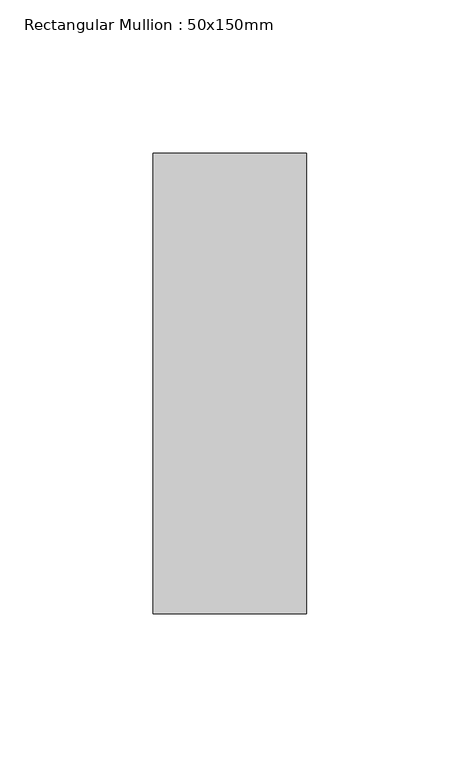
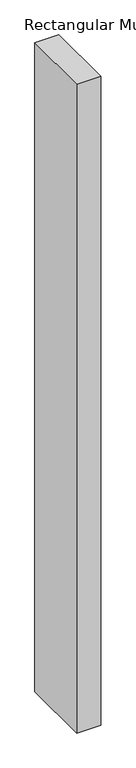
"""IFC4 building model written with IfcOpenShell, lengths in millimetres: member geometry, Rectangular Mullion : 50x150mm."""

import ifcopenshell
import ifcopenshell.guid

model = None  # the IFC model being written
_history = None  # IfcOwnerHistory: only IFC2X3 demands one
_inside = {}  # id of a spatial element -> (the spatial element, [elements in it])
_under = {}  # id of a project, library or spatial element -> (it, [spatial elements below it])
_declared = {}  # id of a project -> (the project, [libraries it declares])
_typed = {}  # id of a type object -> (the type object, [elements of that type])
_made_of = {}  # id of a material, layer set ... -> (it, [elements and type objects made of it])


def new_model(schema):
    """Start an empty IFC model of exactly this schema.

    Asked for "IFC4X3", IfcOpenShell would pick the latest addendum, in which some entities
    have other attributes; the version numbers below select the first issue.
    IFC2X3 requires an IfcOwnerHistory on every rooted entity: one is made here for all.
    """
    global model, _history
    if schema == "IFC4X3":
        model = ifcopenshell.file(schema_version=(4, 3, 0, 0))
    else:
        model = ifcopenshell.file(schema=schema)
    _inside.clear()
    _under.clear()
    _declared.clear()
    _typed.clear()
    _made_of.clear()
    _history = None
    if model.schema == "IFC2X3":
        org = make("IfcOrganization", Name="unknown")
        user = make(
            "IfcPersonAndOrganization",
            ThePerson=make("IfcPerson", FamilyName="unknown"),
            TheOrganization=org,
        )
        app = make(
            "IfcApplication",
            ApplicationDeveloper=org,
            Version="unknown",
            ApplicationFullName="unknown",
            ApplicationIdentifier="unknown",
        )
        _history = make(
            "IfcOwnerHistory",
            OwningUser=user,
            OwningApplication=app,
            ChangeAction="ADDED",
            CreationDate=0,
        )
    return model


def make(cls, **values):
    """One entity of the class cls with the attributes given. An attribute that is None is left unset."""
    return model.create_entity(
        cls, **{name: value for name, value in values.items() if value is not None}
    )


def rooted(cls, **values):
    """An entity with a GlobalId (a new one), such as an element, a storey or a relation."""
    return make(cls, GlobalId=ifcopenshell.guid.new(), OwnerHistory=_history, **values)


def si_unit(unit_type, name, prefix=None):
    """IfcSIUnit, for example si_unit("LENGTHUNIT", "METRE", prefix="MILLI")."""
    return make("IfcSIUnit", UnitType=unit_type, Prefix=prefix, Name=name)


def assignment(units):
    """IfcUnitAssignment: the units of a project."""
    return None if units is None else make("IfcUnitAssignment", Units=units)


def point(xyz):
    """IfcCartesianPoint."""
    return None if xyz is None else make("IfcCartesianPoint", Coordinates=xyz)


def direction(xyz):
    """IfcDirection."""
    return None if xyz is None else make("IfcDirection", DirectionRatios=xyz)


def frame(location, z_axis=None, x_axis=None):
    """IfcAxis2Placement3D, a coordinate frame: its origin and axes. An axis left out is left unset."""
    return make(
        "IfcAxis2Placement3D",
        Location=point(location),
        Axis=direction(z_axis),
        RefDirection=direction(x_axis),
    )


def origin():
    """The frame at (0, 0, 0) with its axes left unset."""
    return frame((0.0, 0.0, 0.0))


def place(relative_to, where):
    """IfcLocalPlacement: puts the frame where relative to a parent placement (None: the world)."""
    return make(
        "IfcLocalPlacement", PlacementRelTo=relative_to, RelativePlacement=where
    )


def context(
    kind, dimensions, precision=None, world=None, true_north=None, identifier=None
):
    """IfcGeometricRepresentationContext, for example the 3D "Model" context."""
    return make(
        "IfcGeometricRepresentationContext",
        ContextIdentifier=identifier,
        ContextType=kind,
        CoordinateSpaceDimension=dimensions,
        Precision=precision,
        WorldCoordinateSystem=world,
        TrueNorth=true_north,
    )


def project(units=None, contexts=None):
    """IfcProject with its units and contexts."""
    return rooted(
        "IfcProject",
        Name="project",
        RepresentationContexts=contexts,
        UnitsInContext=assignment(units),
    )


def spatial(cls, under=None, at=None, **own):
    """A site, building, storey or space (cls), placed at a placement, below another one or the project."""
    s = rooted(cls, ObjectPlacement=at, **own)
    if under is not None:
        _under.setdefault(under.id(), (under, []))[1].append(s)
    return s


def polyline(points):
    """IfcPolyline through the points."""
    return make("IfcPolyline", Points=[point(p) for p in points])


def outline(outer, holes=None, kind="AREA"):
    """IfcArbitraryClosedProfileDef: a profile drawn as a closed curve; with holes, ...WithVoids."""
    if holes is None:
        return make("IfcArbitraryClosedProfileDef", ProfileType=kind, OuterCurve=outer)
    return make(
        "IfcArbitraryProfileDefWithVoids",
        ProfileType=kind,
        OuterCurve=outer,
        InnerCurves=holes,
    )


def extrude(swept, where, along, depth):
    """IfcExtrudedAreaSolid: the profile swept, set in the frame where, extruded along a direction by depth."""
    return make(
        "IfcExtrudedAreaSolid",
        SweptArea=swept,
        Position=where,
        ExtrudedDirection=direction(along),
        Depth=depth,
    )


def shape(context_of_items, identifier, shape_type, items):
    """IfcShapeRepresentation: the items that make up one representation, for example the "Body"."""
    return make(
        "IfcShapeRepresentation",
        ContextOfItems=context_of_items,
        RepresentationIdentifier=identifier,
        RepresentationType=shape_type,
        Items=items,
    )


def source(mapping_origin, context_of_items, identifier, shape_type, items):
    """IfcRepresentationMap: a shape defined once, which mapped items show again and again."""
    return make(
        "IfcRepresentationMap",
        MappingOrigin=mapping_origin,
        MappedRepresentation=shape(context_of_items, identifier, shape_type, items),
    )


def transform(
    local_origin,
    x_axis=None,
    y_axis=None,
    z_axis=None,
    scale=None,
    scale2=None,
    scale3=None,
    uniform=True,
):
    """IfcCartesianTransformationOperator3D, or its non-uniform kind. x_axis, y_axis, z_axis: its Axis1, 2, 3."""
    if uniform:
        return make(
            "IfcCartesianTransformationOperator3D",
            Axis1=direction(x_axis),
            Axis2=direction(y_axis),
            LocalOrigin=point(local_origin),
            Scale=scale,
            Axis3=direction(z_axis),
        )
    return make(
        "IfcCartesianTransformationOperator3DnonUniform",
        Axis1=direction(x_axis),
        Axis2=direction(y_axis),
        LocalOrigin=point(local_origin),
        Scale=scale,
        Axis3=direction(z_axis),
        Scale2=scale2,
        Scale3=scale3,
    )


def mapped(mapping_source, mapping_target):
    """IfcMappedItem: shows the shape of a source again, moved by a transform."""
    return make(
        "IfcMappedItem", MappingSource=mapping_source, MappingTarget=mapping_target
    )


def made_of(thing, what):
    """Note that an element or type object is made of a material, layer set ...; save() writes the relation."""
    if what is not None:
        _made_of.setdefault(what.id(), (what, []))[1].append(thing)
    return thing


def element(
    cls,
    number,
    at=None,
    inside=None,
    cuts=None,
    type_object=None,
    material=None,
    context=None,
    identifier="Body",
    shape_type=None,
    held_by="IfcProductDefinitionShape",
    body=None,
    shapes=None,
    **own,
):
    """One element of the class cls, such as IfcWall. Its Tag is "e" and its number.

    at: its placement. inside: the storey or other place that contains it. cuts: it is an
    opening in that element (IfcRelVoidsElement). A single representation is given by context,
    identifier, shape_type and body (its items); several are given by shapes. held_by: the class
    of the entity that holds the representations. save() writes the other relations.
    """
    e = rooted(cls, Tag="e%d" % number, ObjectPlacement=at, **own)
    if body is not None:
        shapes = [shape(context, identifier, shape_type, body)]
    if shapes is not None:
        e.Representation = make(held_by, Representations=shapes)
    if inside is not None:
        _inside.setdefault(inside.id(), (inside, []))[1].append(e)
    if cuts is not None:
        rooted(
            "IfcRelVoidsElement", RelatingBuildingElement=cuts, RelatedOpeningElement=e
        )
    if type_object is not None:
        _typed.setdefault(type_object.id(), (type_object, []))[1].append(e)
    return made_of(e, material)


def aggregate(whole, parts):
    """IfcRelAggregates: a whole, such as a stair, and the parts it consists of."""
    return rooted("IfcRelAggregates", RelatingObject=whole, RelatedObjects=parts)


def save(model, path):
    """Write the relations noted so far, then the file.

    IfcRelAggregates (storeys below a building ...), IfcRelContainedInSpatialStructure (elements
    in a storey), IfcRelDefinesByType, IfcRelAssociatesMaterial and IfcRelDeclares: one each for
    every whole, place, type object, material and project.
    """
    for whole, parts in _under.values():
        aggregate(whole, parts)
    for where, things in _inside.values():
        rooted(
            "IfcRelContainedInSpatialStructure",
            RelatedElements=things,
            RelatingStructure=where,
        )
    for kind, things in _typed.values():
        rooted("IfcRelDefinesByType", RelatedObjects=things, RelatingType=kind)
    for what, things in _made_of.values():
        rooted("IfcRelAssociatesMaterial", RelatedObjects=things, RelatingMaterial=what)
    for by, libraries in _declared.values():
        rooted("IfcRelDeclares", RelatingContext=by, RelatedDefinitions=libraries)
    model.write(path)


def rectangular_mullion_50x150mm_751a5dca(model_context):
    return source(origin(), model_context, "Body", "SweptSolid", [
        extrude(outline(polyline([(0.0, 75.0), (0.0, -75.0), (-50.0, -75.0), (-50.0, 75.0), (0.0, 75.0)])), frame((0.0, 0.0, -1425.0), z_axis=(0.0, 0.0, 1.0), x_axis=(1.0, 0.0, 0.0)), (0.0, 0.0, 1.0), 1425.0),
    ])


if __name__ == "__main__":
    model = new_model("IFC4")
    model_context = context("Model", 3, world=origin())
    ifc_project = project(units=[si_unit("LENGTHUNIT", "METRE", prefix="MILLI")], contexts=[model_context])
    site = spatial("IfcSite", under=ifc_project)
    building = spatial("IfcBuilding", under=site)
    placement = place(None, origin())
    rectangular_mullion_50x150mm_shape = rectangular_mullion_50x150mm_751a5dca(model_context)
    element("IfcMember", 1, ObjectType="Rectangular Mullion : 50x150mm", at=placement, inside=building, context=model_context, shape_type="MappedRepresentation", body=[
        mapped(rectangular_mullion_50x150mm_shape, transform((0.0, 0.0, 0.0), x_axis=(1.0, 0.0, 0.0), y_axis=(0.0, 1.0, 0.0), z_axis=(0.0, 0.0, 1.0))),
    ])
    save(model, "model.ifc")

# Revit data of these elements
# Type "Rectangular Mullion : 50x150mm"
#   Keynote = "H11"
#   built-in parameter 1007304 = 0.492126 (stored number, unit not read)
#   built-in parameter 1007301 = 0.082021 (stored number, unit not read)
#   built-in parameter 1007300 = 0.082021 (stored number, unit not read)
# Element 1 (IfcMember, "Rectangular Mullion : 50x150mm")
#   Materials on its faces: "Aluminium"
# Materials
#   "Aluminium": class "Metal", colour RGB 247 247 247, transparency 0, Description = "Aluminium 6061", Cost = 0
